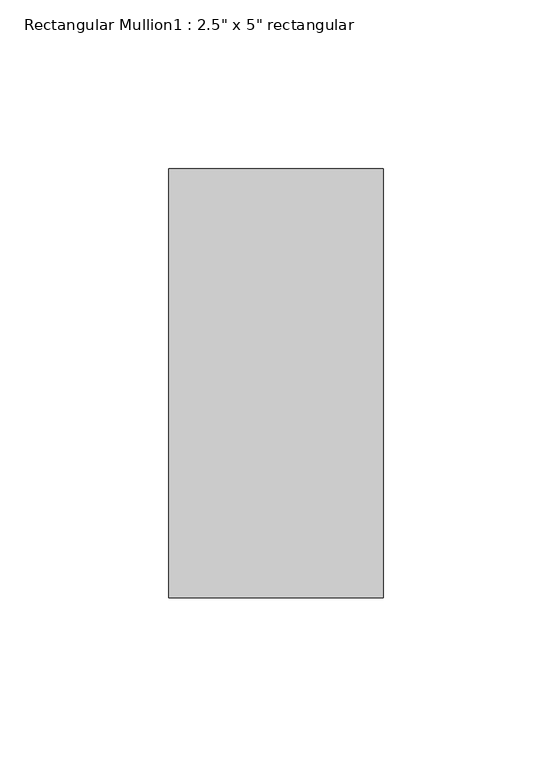
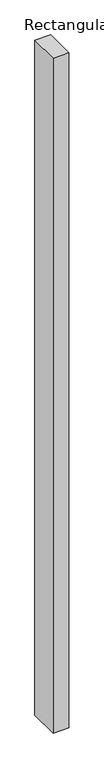
"""IFC4 building model written with IfcOpenShell, lengths in millimetres: member geometry."""

import ifcopenshell
import ifcopenshell.guid

model = None  # the IFC model being written
_history = None  # IfcOwnerHistory: only IFC2X3 demands one
_inside = {}  # id of a spatial element -> (the spatial element, [elements in it])
_under = {}  # id of a project, library or spatial element -> (it, [spatial elements below it])
_declared = {}  # id of a project -> (the project, [libraries it declares])
_typed = {}  # id of a type object -> (the type object, [elements of that type])
_made_of = {}  # id of a material, layer set ... -> (it, [elements and type objects made of it])


def new_model(schema):
    """Start an empty IFC model of exactly this schema.

    Asked for "IFC4X3", IfcOpenShell would pick the latest addendum, in which some entities
    have other attributes; the version numbers below select the first issue.
    IFC2X3 requires an IfcOwnerHistory on every rooted entity: one is made here for all.
    """
    global model, _history
    if schema == "IFC4X3":
        model = ifcopenshell.file(schema_version=(4, 3, 0, 0))
    else:
        model = ifcopenshell.file(schema=schema)
    _inside.clear()
    _under.clear()
    _declared.clear()
    _typed.clear()
    _made_of.clear()
    _history = None
    if model.schema == "IFC2X3":
        org = make("IfcOrganization", Name="unknown")
        user = make(
            "IfcPersonAndOrganization",
            ThePerson=make("IfcPerson", FamilyName="unknown"),
            TheOrganization=org,
        )
        app = make(
            "IfcApplication",
            ApplicationDeveloper=org,
            Version="unknown",
            ApplicationFullName="unknown",
            ApplicationIdentifier="unknown",
        )
        _history = make(
            "IfcOwnerHistory",
            OwningUser=user,
            OwningApplication=app,
            ChangeAction="ADDED",
            CreationDate=0,
        )
    return model


def make(cls, **values):
    """One entity of the class cls with the attributes given. An attribute that is None is left unset."""
    return model.create_entity(
        cls, **{name: value for name, value in values.items() if value is not None}
    )


def rooted(cls, **values):
    """An entity with a GlobalId (a new one), such as an element, a storey or a relation."""
    return make(cls, GlobalId=ifcopenshell.guid.new(), OwnerHistory=_history, **values)


def si_unit(unit_type, name, prefix=None):
    """IfcSIUnit, for example si_unit("LENGTHUNIT", "METRE", prefix="MILLI")."""
    return make("IfcSIUnit", UnitType=unit_type, Prefix=prefix, Name=name)


def assignment(units):
    """IfcUnitAssignment: the units of a project."""
    return None if units is None else make("IfcUnitAssignment", Units=units)


def point(xyz):
    """IfcCartesianPoint."""
    return None if xyz is None else make("IfcCartesianPoint", Coordinates=xyz)


def direction(xyz):
    """IfcDirection."""
    return None if xyz is None else make("IfcDirection", DirectionRatios=xyz)


def frame(location, z_axis=None, x_axis=None):
    """IfcAxis2Placement3D, a coordinate frame: its origin and axes. An axis left out is left unset."""
    return make(
        "IfcAxis2Placement3D",
        Location=point(location),
        Axis=direction(z_axis),
        RefDirection=direction(x_axis),
    )


def origin():
    """The frame at (0, 0, 0) with its axes left unset."""
    return frame((0.0, 0.0, 0.0))


def place(relative_to, where):
    """IfcLocalPlacement: puts the frame where relative to a parent placement (None: the world)."""
    return make(
        "IfcLocalPlacement", PlacementRelTo=relative_to, RelativePlacement=where
    )


def context(
    kind, dimensions, precision=None, world=None, true_north=None, identifier=None
):
    """IfcGeometricRepresentationContext, for example the 3D "Model" context."""
    return make(
        "IfcGeometricRepresentationContext",
        ContextIdentifier=identifier,
        ContextType=kind,
        CoordinateSpaceDimension=dimensions,
        Precision=precision,
        WorldCoordinateSystem=world,
        TrueNorth=true_north,
    )


def project(units=None, contexts=None):
    """IfcProject with its units and contexts."""
    return rooted(
        "IfcProject",
        Name="project",
        RepresentationContexts=contexts,
        UnitsInContext=assignment(units),
    )


def spatial(cls, under=None, at=None, **own):
    """A site, building, storey or space (cls), placed at a placement, below another one or the project."""
    s = rooted(cls, ObjectPlacement=at, **own)
    if under is not None:
        _under.setdefault(under.id(), (under, []))[1].append(s)
    return s


def polyline(points):
    """IfcPolyline through the points."""
    return make("IfcPolyline", Points=[point(p) for p in points])


def outline(outer, holes=None, kind="AREA"):
    """IfcArbitraryClosedProfileDef: a profile drawn as a closed curve; with holes, ...WithVoids."""
    if holes is None:
        return make("IfcArbitraryClosedProfileDef", ProfileType=kind, OuterCurve=outer)
    return make(
        "IfcArbitraryProfileDefWithVoids",
        ProfileType=kind,
        OuterCurve=outer,
        InnerCurves=holes,
    )


def extrude(swept, where, along, depth):
    """IfcExtrudedAreaSolid: the profile swept, set in the frame where, extruded along a direction by depth."""
    return make(
        "IfcExtrudedAreaSolid",
        SweptArea=swept,
        Position=where,
        ExtrudedDirection=direction(along),
        Depth=depth,
    )


def shape(context_of_items, identifier, shape_type, items):
    """IfcShapeRepresentation: the items that make up one representation, for example the "Body"."""
    return make(
        "IfcShapeRepresentation",
        ContextOfItems=context_of_items,
        RepresentationIdentifier=identifier,
        RepresentationType=shape_type,
        Items=items,
    )


def source(mapping_origin, context_of_items, identifier, shape_type, items):
    """IfcRepresentationMap: a shape defined once, which mapped items show again and again."""
    return make(
        "IfcRepresentationMap",
        MappingOrigin=mapping_origin,
        MappedRepresentation=shape(context_of_items, identifier, shape_type, items),
    )


def transform(
    local_origin,
    x_axis=None,
    y_axis=None,
    z_axis=None,
    scale=None,
    scale2=None,
    scale3=None,
    uniform=True,
):
    """IfcCartesianTransformationOperator3D, or its non-uniform kind. x_axis, y_axis, z_axis: its Axis1, 2, 3."""
    if uniform:
        return make(
            "IfcCartesianTransformationOperator3D",
            Axis1=direction(x_axis),
            Axis2=direction(y_axis),
            LocalOrigin=point(local_origin),
            Scale=scale,
            Axis3=direction(z_axis),
        )
    return make(
        "IfcCartesianTransformationOperator3DnonUniform",
        Axis1=direction(x_axis),
        Axis2=direction(y_axis),
        LocalOrigin=point(local_origin),
        Scale=scale,
        Axis3=direction(z_axis),
        Scale2=scale2,
        Scale3=scale3,
    )


def mapped(mapping_source, mapping_target):
    """IfcMappedItem: shows the shape of a source again, moved by a transform."""
    return make(
        "IfcMappedItem", MappingSource=mapping_source, MappingTarget=mapping_target
    )


def made_of(thing, what):
    """Note that an element or type object is made of a material, layer set ...; save() writes the relation."""
    if what is not None:
        _made_of.setdefault(what.id(), (what, []))[1].append(thing)
    return thing


def element(
    cls,
    number,
    at=None,
    inside=None,
    cuts=None,
    type_object=None,
    material=None,
    context=None,
    identifier="Body",
    shape_type=None,
    held_by="IfcProductDefinitionShape",
    body=None,
    shapes=None,
    **own,
):
    """One element of the class cls, such as IfcWall. Its Tag is "e" and its number.

    at: its placement. inside: the storey or other place that contains it. cuts: it is an
    opening in that element (IfcRelVoidsElement). A single representation is given by context,
    identifier, shape_type and body (its items); several are given by shapes. held_by: the class
    of the entity that holds the representations. save() writes the other relations.
    """
    e = rooted(cls, Tag="e%d" % number, ObjectPlacement=at, **own)
    if body is not None:
        shapes = [shape(context, identifier, shape_type, body)]
    if shapes is not None:
        e.Representation = make(held_by, Representations=shapes)
    if inside is not None:
        _inside.setdefault(inside.id(), (inside, []))[1].append(e)
    if cuts is not None:
        rooted(
            "IfcRelVoidsElement", RelatingBuildingElement=cuts, RelatedOpeningElement=e
        )
    if type_object is not None:
        _typed.setdefault(type_object.id(), (type_object, []))[1].append(e)
    return made_of(e, material)


def aggregate(whole, parts):
    """IfcRelAggregates: a whole, such as a stair, and the parts it consists of."""
    return rooted("IfcRelAggregates", RelatingObject=whole, RelatedObjects=parts)


def save(model, path):
    """Write the relations noted so far, then the file.

    IfcRelAggregates (storeys below a building ...), IfcRelContainedInSpatialStructure (elements
    in a storey), IfcRelDefinesByType, IfcRelAssociatesMaterial and IfcRelDeclares: one each for
    every whole, place, type object, material and project.
    """
    for whole, parts in _under.values():
        aggregate(whole, parts)
    for where, things in _inside.values():
        rooted(
            "IfcRelContainedInSpatialStructure",
            RelatedElements=things,
            RelatingStructure=where,
        )
    for kind, things in _typed.values():
        rooted("IfcRelDefinesByType", RelatedObjects=things, RelatingType=kind)
    for what, things in _made_of.values():
        rooted("IfcRelAssociatesMaterial", RelatedObjects=things, RelatingMaterial=what)
    for by, libraries in _declared.values():
        rooted("IfcRelDeclares", RelatingContext=by, RelatedDefinitions=libraries)
    model.write(path)


def member_ef0f639d(model_context):
    return source(origin(), model_context, "Body", "SweptSolid", [
        extrude(outline(polyline([(0.0, 63.5), (0.0, -63.5), (-63.5, -63.5), (-63.5, 63.5), (0.0, 63.5)])), frame((0.0, 0.0, -2884.17), z_axis=(0.0, 0.0, 1.0), x_axis=(1.0, 0.0, 0.0)), (0.0, 0.0, 1.0), 2884.17),
    ])


if __name__ == "__main__":
    model = new_model("IFC4")
    model_context = context("Model", 3, world=origin())
    ifc_project = project(units=[si_unit("LENGTHUNIT", "METRE", prefix="MILLI")], contexts=[model_context])
    site = spatial("IfcSite", under=ifc_project)
    building = spatial("IfcBuilding", under=site)
    placement = place(None, origin())
    member_shape = member_ef0f639d(model_context)
    element("IfcMember", 1, ObjectType="Rectangular Mullion1 : 2.5\" x 5\" rectangular", at=placement, inside=building, context=model_context, shape_type="MappedRepresentation", body=[
        mapped(member_shape, transform((0.0, 0.0, 0.0), x_axis=(1.0, 0.0, 0.0), y_axis=(0.0, 1.0, 0.0), z_axis=(0.0, 0.0, 1.0))),
    ])
    save(model, "model.ifc")

# Revit data of these elements
# Type "Rectangular Mullion1 : 2.5\" x 5\" rectangular"
#   built-in parameter 1007304 = 0.416667 (stored number, unit not read)
#   built-in parameter 1007301 = 0.104167 (stored number, unit not read)
#   built-in parameter 1007300 = 0.104167 (stored number, unit not read)
# Element 1 (IfcMember, "Rectangular Mullion1 : 2.5\" x 5\" rectangular")
#   Materials on its faces: "support-frame"
# Materials
#   "support-frame": class "Unassigned", colour RGB 233 233 233, transparency 0, Cost = 0
